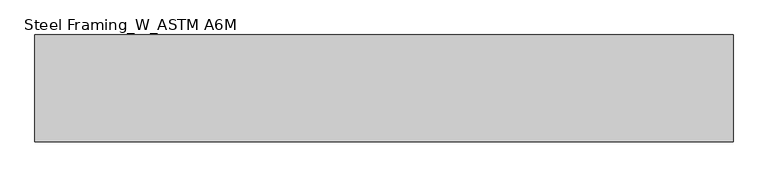
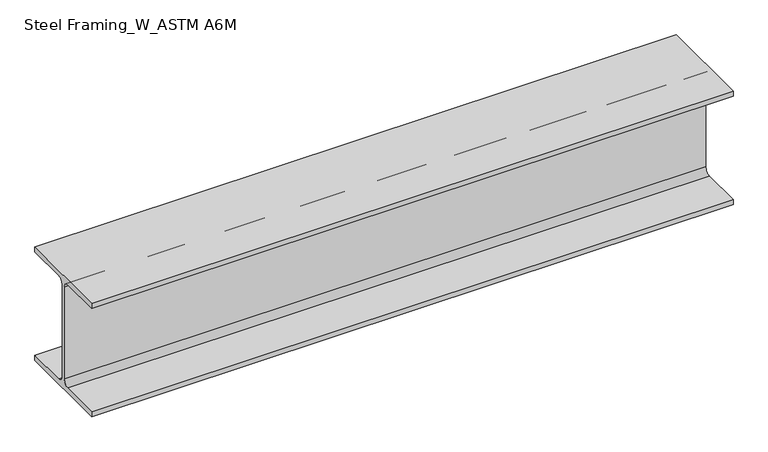
"""IFC4 building model written with IfcOpenShell, lengths in millimetres: beam geometry, Steel Framing_W_ASTM A6M : H_SB_AR_S02_W250x49.1_G5."""

from ifc_helpers import new_model, si_unit, point, frame, frame_2d, origin, place, context, project, spatial, polyline, circle_curve, trimmed, segment, composite_curve, outline, extrude, source, transform, mapped, element, save


def steel_framing_w_astm_a6m_7f0d9279(model_context):
    return source(origin(), model_context, "Body", "SweptSolid", [
        extrude(outline(composite_curve([segment(polyline([(101.0, -112.5), (101.0, -123.5), (-101.0, -123.5), (-101.0, -112.5), (-16.385, -112.5)]), True, "CONTINUOUS"), segment(trimmed(circle_curve(frame_2d((-16.385, -99.8)), 12.7), [point((-16.385, -112.5))], [point((-3.685, -99.8))], True, "CARTESIAN"), True, "CONTINUOUS"), segment(polyline([(-3.685, -99.8), (-3.685, 99.8)]), True, "CONTINUOUS"), segment(trimmed(circle_curve(frame_2d((-16.385, 99.8)), 12.7), [point((-3.685, 99.8))], [point((-16.385, 112.5))], True, "CARTESIAN"), True, "CONTINUOUS"), segment(polyline([(-16.385, 112.5), (-101.0, 112.5), (-101.0, 123.5), (101.0, 123.5), (101.0, 112.5), (16.385, 112.5)]), True, "CONTINUOUS"), segment(trimmed(circle_curve(frame_2d((16.385, 99.8)), 12.7), [point((16.385, 112.5))], [point((3.685, 99.8))], True, "CARTESIAN"), True, "CONTINUOUS"), segment(polyline([(3.685, 99.8), (3.685, -99.8)]), True, "CONTINUOUS"), segment(trimmed(circle_curve(frame_2d((16.385, -99.8)), 12.7), [point((3.685, -99.8))], [point((16.385, -112.5))], True, "CARTESIAN"), True, "CONTINUOUS"), segment(polyline([(16.385, -112.5), (101.0, -112.5)]), True, "CONTINUOUS")], self_intersect=False)), frame((-503.8, 0.0, 0.0), z_axis=(1.0, 0.0, 0.0), x_axis=(0.0, 1.0, 0.0)), (0.0, 0.0, 1.0), 1320.8),
    ])


if __name__ == "__main__":
    model = new_model("IFC4")
    model_context = context("Model", 3, world=origin())
    ifc_project = project(units=[si_unit("LENGTHUNIT", "METRE", prefix="MILLI")], contexts=[model_context])
    site = spatial("IfcSite", under=ifc_project)
    building = spatial("IfcBuilding", under=site)
    placement = place(None, origin())
    steel_framing_w_astm_a6m_shape = steel_framing_w_astm_a6m_7f0d9279(model_context)
    element("IfcBeam", 1, ObjectType="Steel Framing_W_ASTM A6M : H_SB_AR_S02_W250x49.1_G5", at=placement, inside=building, context=model_context, shape_type="MappedRepresentation", body=[
        mapped(steel_framing_w_astm_a6m_shape, transform((0.0, 0.0, 0.0), x_axis=(1.0, 0.0, 0.0), y_axis=(0.0, 1.0, 0.0), z_axis=(0.0, 0.0, 1.0))),
    ])
    save(model, "model.ifc")

# Revit data of these elements
# Type "Steel Framing_W_ASTM A6M : H_SB_AR_S02_W250x49.1_G5"
#   Type Mark = "G5"
#   Section Name Key = "W10x33"
#   Width = 20.2 cm
#   Web Thickness = 0.737 cm
#   Web Fillet = 1.27 cm
#   Warping Constant = 212000.0 cm⁶
#   Torsional Moment of Inertia = 24.30 cm⁴
#   Section Area = 62.6 cm²
#   Plastic Modulus weak axis = 229.0 cm³
#   Plastic Modulus strong axis = 636.0 cm³
#   Perimeter = 1.27 m²/m
#   Nominal Weight = 49.10 kgf/m
#   Moment of Inertia weak axis = 1520.00 cm⁴
#   Moment of Inertia strong axis = 7120.00 cm⁴
#   Height = 24.7 cm
#   Flange Thickness = 1.1 cm
#   Elastic Modulus weak axis = 151.0 cm³
#   Elastic Modulus strong axis = 574.0 cm³
#   Centroid Vertical = 12.35 cm
#   Centroid Horizontal = 10.1 cm
#   Length [instance default] = 1500 mm
#   Structural Material [instance default] = Steel, 45-345
#   Bolt Spacing = 0
#   Assembly Code = ""
# Element 1 (IfcBeam, "Steel Framing_W_ASTM A6M : H_SB_AR_S02_W250x49.1_G5")
#   Materials on its faces: "Steel, 45-345"
# Materials
#   "Steel, 45-345": class "Metal", colour RGB 189 187 185, transparency 0, Description = "Steel 345 MPa", Cost = 0
